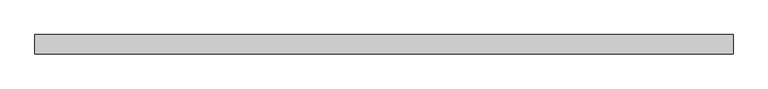
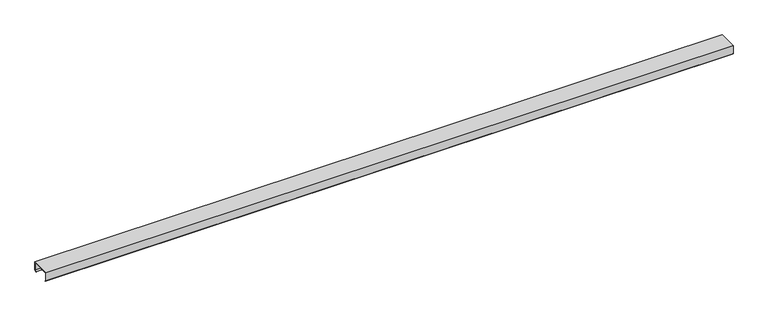
"""IFC4 building model written with IfcOpenShell, lengths in millimetres: proxy geometry, Generic Models 7:Generic Models 1:1:Generic Models 1:1 : Generic Models 7:Generic Models 1:337419:9 : Generic Models 7:Generic Models 1:1:Generic Models 1:1 : Generic Models 7:Generic Models 1:337419:306201."""

from ifc_helpers import new_model, si_unit, frame, origin, place, context, project, spatial, polyline, outline, extrude, source, transform, mapped, element, save


def generic_models_0c1aad58(model_context):
    return source(origin(), model_context, "Body", "SweptSolid", [
        extrude(outline(polyline([(-579000.6913841, 6128.940625), (-578797.4913841, 6128.940625), (-578797.4913841, 6040.040625), (-578812.0845307, 6027.7955211), (-578813.8702751, 6029.9236883), (-578800.2695091, 6041.336086), (-578800.2695091, 6126.1625), (-578997.9132591, 6126.1625), (-578997.9132591, 6041.336086), (-578984.3124931, 6029.9236883), (-578986.0982375, 6027.7955211), (-579000.6913841, 6040.040625), (-579000.6913841, 6128.940625)])), frame((565582.1867239, 0.0, 0.0), z_axis=(1.0, 0.0, 0.0), x_axis=(0.0, 1.0, 0.0)), (0.0, 0.0, 1.0), 7315.2),
    ])


if __name__ == "__main__":
    model = new_model("IFC4")
    model_context = context("Model", 3, world=origin())
    ifc_project = project(units=[si_unit("LENGTHUNIT", "METRE", prefix="MILLI")], contexts=[model_context])
    site = spatial("IfcSite", under=ifc_project)
    building = spatial("IfcBuilding", under=site)
    placement = place(None, origin())
    generic_models_shape = generic_models_0c1aad58(model_context)
    element("IfcBuildingElementProxy", 1, Name="Generic Models 7:Generic Models 1:1:Generic Models 1:1 : Generic Models 7:Generic Models 1:337419:9 : Generic Models 7:Generic Models 1:1:Generic Models 1:1 : Generic Models 7:Generic Models 1:337419:306201", ObjectType="Generic Models 7:Generic Models 1:1:Generic Models 1:1 : Generic Models 7:Generic Models 1:337419:9 : Generic Models 7:Generic Models 1:1:Generic Models 1:1 : Generic Models 7:Generic Models 1:337419:306201", at=placement, inside=building, context=model_context, shape_type="MappedRepresentation", body=[
        mapped(generic_models_shape, transform((0.0, 0.0, 0.0), x_axis=(1.0, 0.0, 0.0), y_axis=(0.0, 1.0, 0.0), z_axis=(0.0, 0.0, 1.0))),
    ])
    save(model, "model.ifc")

# Revit data of these elements
# Type "Generic Models 7:Generic Models 1:1:Generic Models 1:1 : Generic Models 7:Generic Models 1:337419:9 : Generic Models 7:Generic Models 1:1:Generic Models 1:1 : Generic Models 7:Generic Models 1:337419:306201"
#   NameOverride = "Generic Models 7:Generic Models 1:1:Generic Models 1:1 : Generic Models 7:Generic Models 1:337419:306201"
#   ObjectTypeOverride = "Generic Models 1:1 : Generic Models 7:Generic Models 1:337419"
#   Reference = "Generic Models 1"
#   Tag = "306201"
# Element 1 (IfcBuildingElementProxy, "Generic Models 7:Generic Models 1:1:Generic Models 1:1 : Generic Models 7:Generic Models 1:337419:9 : Generic Models 7:Generic Models 1:1:Generic Models 1:1 : Generic Models 7:Generic Models 1:337419:306201")
#   Materials on its faces: "CEE' SECTION (8.0x3.5C - SEE STRUCT. DWGS)"
# Materials
#   "CEE' SECTION (8.0x3.5C - SEE STRUCT. DWGS)": class "Unassigned", colour RGB 210 209 208, transparency 0, Keynote = "M05121300.02", Cost = 0
